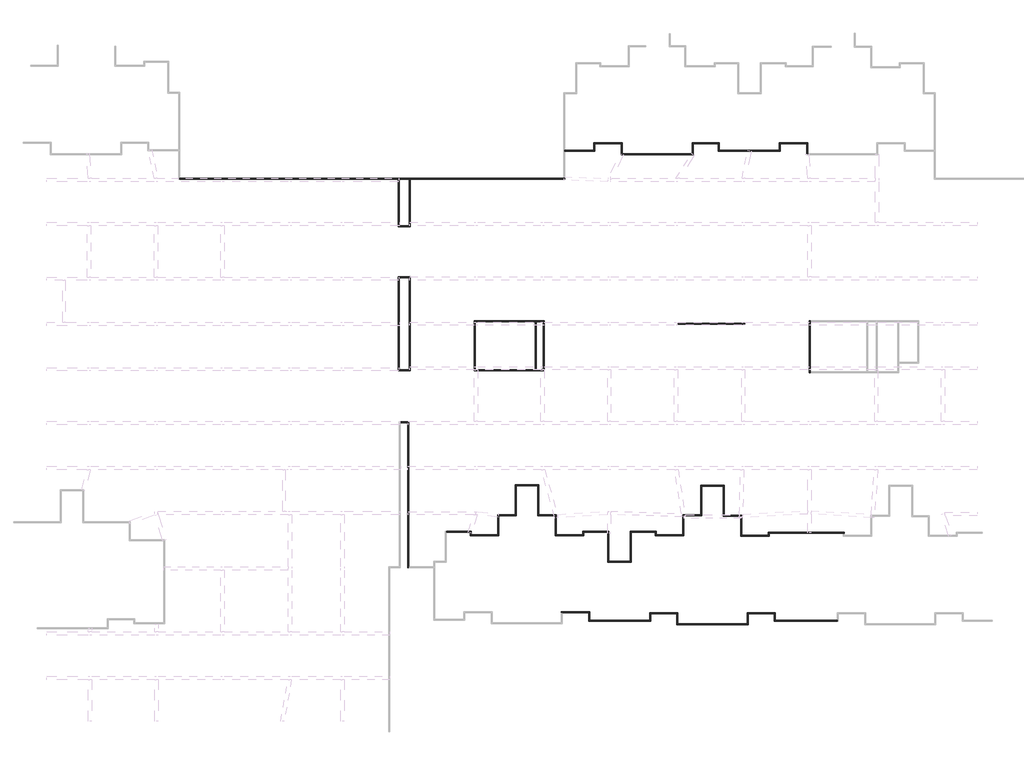
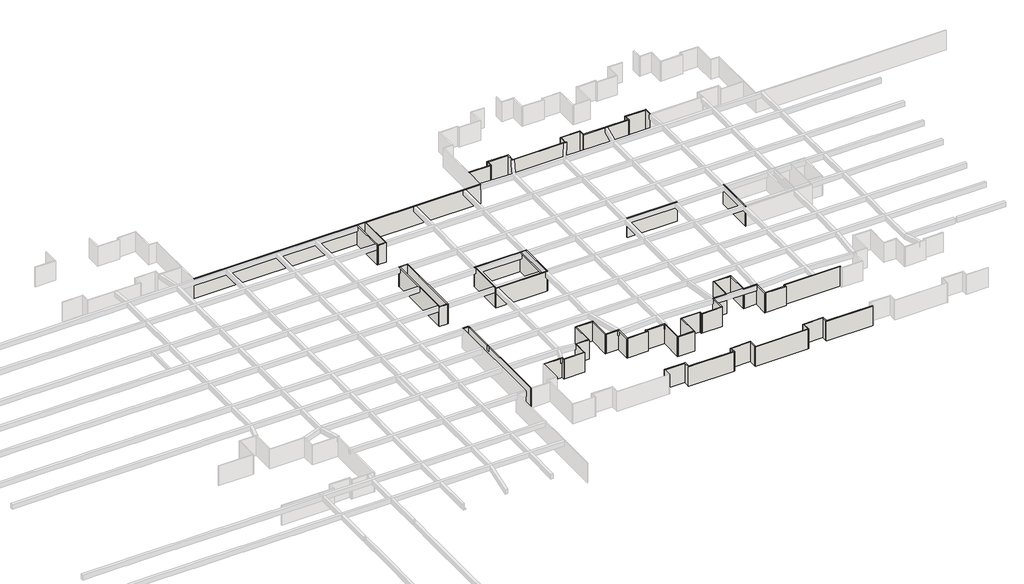
# One storey, part 5 of 16: 69 walls.
"""IFC4 building model written with IfcOpenShell, lengths in millimetres."""

from ifc_helpers import new_model, si_unit, origin, origin_with_axes, place, context, project, spatial, polyline, outline, extrude, faceted_brep, element, save

model = new_model("IFC4")

# Units and contexts
model_context = context("Model", 3, world=origin())
ifc_project = project(units=[si_unit("LENGTHUNIT", "METRE", prefix="MILLI")], contexts=[model_context])

# Site, building, storey
site = spatial("IfcSite", under=ifc_project)
building = spatial("IfcBuilding", under=site)
storey = spatial("IfcBuildingStorey", under=building, Name="户型图", Elevation=0.0)

# Walls
placement = place(None, origin())
element("IfcWall", 1, ObjectType="所有墙体", at=placement, inside=storey, context=model_context, shape_type="Brep", body=[
    faceted_brep([(305726.5285699, -132365.1471774, 0.0), (331943.757676, -132365.1471774, 0.0), (332063.757676, -132365.1471774, 0.0), (333243.7576761, -132365.1471774, 0.0), (333363.7576761, -132365.1471774, 0.0), (351926.5285699, -132365.1471774, 0.0), (351926.5285699, -132365.1471774, 3300.0), (333363.7576761, -132365.1471774, 3300.0), (333243.7576761, -132365.1471774, 3300.0), (332063.757676, -132365.1471774, 3300.0), (331943.757676, -132365.1471774, 3300.0), (305726.5285699, -132365.1471774, 3300.0), (305726.5285699, -132245.1471774, 0.0), (305726.5285699, -132245.1471774, 3300.0), (351806.5285699, -132245.1471774, 3300.0), (351926.5285699, -132245.1471774, 3300.0), (351926.5285699, -132245.1471774, 0.0), (351806.5285699, -132245.1471774, 0.0)], [[[0, 1, 2, 3, 4, 5, 6, 7, 8, 9, 10, 11]], [[12, 13, 14, 15, 16, 17]], [[5, 4, 3, 2, 1, 0, 12, 17, 16]], [[11, 10, 9, 8, 7, 6, 15, 14, 13]], [[0, 11, 13, 12]], [[6, 5, 16, 15]]]),
])
element("IfcWall", 2, ObjectType="所有墙体", at=placement, inside=storey, context=model_context, shape_type="Brep", body=[
    faceted_brep([(381017.0370116, -129335.4591871, 0.0), (381017.0370116, -128039.1416737, 0.0), (381017.0370116, -128039.1416737, 3300.0), (381017.0370116, -129335.4591871, 3300.0), (380897.0370116, -129335.4591871, 0.0), (380897.0370116, -129335.4591871, 3300.0), (380897.0370116, -128159.1416737, 3300.0), (380897.0370116, -128039.1416737, 3300.0), (380897.0370116, -128039.1416737, 0.0), (380897.0370116, -128159.1416737, 0.0)], [[[0, 1, 2, 3]], [[4, 5, 6, 7, 8, 9]], [[1, 0, 4, 9, 8]], [[3, 2, 7, 6, 5]], [[0, 3, 5, 4]], [[2, 1, 8, 7]]]),
])
element("IfcWall", 3, ObjectType="所有墙体", at=placement, inside=storey, context=model_context, shape_type="Brep", body=[
    faceted_brep([(380897.0370116, -128039.1416737, 0.0), (377598.9141674, -128039.1416737, 0.0), (377598.9141674, -128039.1416737, 3300.0), (380897.0370116, -128039.1416737, 3300.0), (380897.0370116, -128159.1416737, 0.0), (380897.0370116, -128159.1416737, 3300.0), (377718.9141674, -128159.1416737, 3300.0), (377598.9141674, -128159.1416737, 3300.0), (377598.9141674, -128159.1416737, 0.0), (377718.9141674, -128159.1416737, 0.0)], [[[0, 1, 2, 3]], [[4, 5, 6, 7, 8, 9]], [[1, 0, 4, 9, 8]], [[3, 2, 7, 6, 5]], [[0, 3, 5, 4]], [[2, 1, 8, 7]]]),
])
element("IfcWall", 4, ObjectType="所有墙体", at=placement, inside=storey, context=model_context, shape_type="Brep", body=[
    faceted_brep([(377598.9141674, -128159.1416737, 0.0), (377598.9141674, -128941.8026441, 0.0), (377598.9141674, -129061.8026441, 0.0), (377598.9141674, -129061.8026441, 3300.0), (377598.9141674, -128941.8026441, 3300.0), (377598.9141674, -128159.1416737, 3300.0), (377718.9141674, -128159.1416737, 0.0), (377718.9141674, -128159.1416737, 3300.0), (377718.9141674, -129061.8026441, 3300.0), (377718.9141674, -129061.8026441, 0.0)], [[[0, 1, 2, 3, 4, 5]], [[6, 7, 8, 9]], [[2, 1, 0, 6, 9]], [[5, 4, 3, 8, 7]], [[0, 5, 7, 6]], [[3, 2, 9, 8]]]),
])
element("IfcWall", 5, ObjectType="所有墙体", at=placement, inside=storey, context=model_context, shape_type="Brep", body=[
    faceted_brep([(377598.9141674, -128941.8026441, 0.0), (370417.9023455, -128941.8026441, 0.0), (370297.9023455, -128941.8026441, 0.0), (370297.9023455, -128941.8026441, 3300.0), (370417.9023455, -128941.8026441, 3300.0), (377598.9141674, -128941.8026441, 3300.0), (377598.9141674, -129061.8026441, 0.0), (377598.9141674, -129061.8026441, 3300.0), (370297.9023455, -129061.8026441, 3300.0), (370297.9023455, -129061.8026441, 0.0)], [[[0, 1, 2, 3, 4, 5]], [[6, 7, 8, 9]], [[2, 1, 0, 6, 9]], [[5, 4, 3, 8, 7]], [[0, 5, 7, 6]], [[3, 2, 9, 8]]]),
])
element("IfcWall", 6, ObjectType="所有墙体", at=placement, inside=storey, context=model_context, shape_type="Brep", body=[
    faceted_brep([(370417.9023455, -128941.8026441, 0.0), (370417.9023455, -128039.1416737, 0.0), (370417.9023455, -128039.1416737, 3300.0), (370417.9023455, -128941.8026441, 3300.0), (370297.9023455, -128941.8026441, 0.0), (370297.9023455, -128941.8026441, 3300.0), (370297.9023455, -128159.1416737, 3300.0), (370297.9023455, -128039.1416737, 3300.0), (370297.9023455, -128039.1416737, 0.0), (370297.9023455, -128159.1416737, 0.0)], [[[0, 1, 2, 3]], [[4, 5, 6, 7, 8, 9]], [[1, 0, 4, 9, 8]], [[3, 2, 7, 6, 5]], [[0, 3, 5, 4]], [[2, 1, 8, 7]]]),
])
element("IfcWall", 7, ObjectType="所有墙体", at=placement, inside=storey, context=model_context, shape_type="Brep", body=[
    faceted_brep([(370297.9023455, -128039.1416737, 0.0), (367198.9076923, -128039.1416737, 0.0), (367198.9076923, -128039.1416737, 3300.0), (370297.9023455, -128039.1416737, 3300.0), (370297.9023455, -128159.1416737, 0.0), (370297.9023455, -128159.1416737, 3300.0), (367318.9076923, -128159.1416737, 3300.0), (367198.9076923, -128159.1416737, 3300.0), (367198.9076923, -128159.1416737, 0.0), (367318.9076923, -128159.1416737, 0.0)], [[[0, 1, 2, 3]], [[4, 5, 6, 7, 8, 9]], [[1, 0, 4, 9, 8]], [[3, 2, 7, 6, 5]], [[0, 3, 5, 4]], [[2, 1, 8, 7]]]),
])
element("IfcWall", 8, ObjectType="所有墙体", at=placement, inside=storey, context=model_context, shape_type="Brep", body=[
    faceted_brep([(367198.9076923, -128159.1416737, 0.0), (367198.9076923, -129335.4591871, 0.0), (367198.9076923, -129455.4591871, 0.0), (367198.9076923, -129455.4591871, 3300.0), (367198.9076923, -129335.4591871, 3300.0), (367198.9076923, -128159.1416737, 3300.0), (367318.9076923, -128159.1416737, 0.0), (367318.9076923, -128159.1416737, 3300.0), (367318.9076923, -129455.4591871, 3300.0), (367318.9076923, -129455.4591871, 0.0)], [[[0, 1, 2, 3, 4, 5]], [[6, 7, 8, 9]], [[2, 1, 0, 6, 9]], [[5, 4, 3, 8, 7]], [[0, 5, 7, 6]], [[3, 2, 9, 8]]]),
])
element("IfcWall", 9, ObjectType="所有墙体", at=placement, inside=storey, context=model_context, shape_type="Brep", body=[
    faceted_brep([(367198.9076923, -129335.4591871, 0.0), (358817.8429758, -129335.4591871, 0.0), (358697.8429758, -129335.4591871, 0.0), (358697.8429758, -129335.4591871, 3300.0), (358817.8429758, -129335.4591871, 3300.0), (367198.9076923, -129335.4591871, 3300.0), (367198.9076923, -129455.4591871, 0.0), (367198.9076923, -129455.4591871, 3300.0), (358697.8429758, -129455.4591871, 3300.0), (358697.8429758, -129455.4591871, 0.0)], [[[0, 1, 2, 3, 4, 5]], [[6, 7, 8, 9]], [[2, 1, 0, 6, 9]], [[5, 4, 3, 8, 7]], [[0, 5, 7, 6]], [[3, 2, 9, 8]]]),
])
element("IfcWall", 10, ObjectType="所有墙体", at=placement, inside=storey, context=model_context, shape_type="Brep", body=[
    faceted_brep([(358817.8429758, -129335.4591871, 0.0), (358817.8429758, -128039.1416737, 0.0), (358817.8429758, -128039.1416737, 3300.0), (358817.8429758, -129335.4591871, 3300.0), (358697.8429758, -129335.4591871, 0.0), (358697.8429758, -129335.4591871, 3300.0), (358697.8429758, -128159.1416737, 3300.0), (358697.8429758, -128039.1416737, 3300.0), (358697.8429758, -128039.1416737, 0.0), (358697.8429758, -128159.1416737, 0.0)], [[[0, 1, 2, 3]], [[4, 5, 6, 7, 8, 9]], [[1, 0, 4, 9, 8]], [[3, 2, 7, 6, 5]], [[0, 3, 5, 4]], [[2, 1, 8, 7]]]),
])
element("IfcWall", 11, ObjectType="所有墙体", at=placement, inside=storey, context=model_context, shape_type="Brep", body=[
    faceted_brep([(358697.8429758, -128039.1416737, 0.0), (355398.9003454, -128039.1416737, 0.0), (355398.9003454, -128039.1416737, 3300.0), (358697.8429758, -128039.1416737, 3300.0), (358697.8429758, -128159.1416737, 0.0), (358697.8429758, -128159.1416737, 3300.0), (355518.9003454, -128159.1416737, 3300.0), (355398.9003454, -128159.1416737, 3300.0), (355398.9003454, -128159.1416737, 0.0), (355518.9003454, -128159.1416737, 0.0)], [[[0, 1, 2, 3]], [[4, 5, 6, 7, 8, 9]], [[1, 0, 4, 9, 8]], [[3, 2, 7, 6, 5]], [[0, 3, 5, 4]], [[2, 1, 8, 7]]]),
])
element("IfcWall", 12, ObjectType="所有墙体", at=placement, inside=storey, context=model_context, shape_type="Brep", body=[
    faceted_brep([(355398.9003454, -128159.1416737, 0.0), (355398.9003454, -128941.8026441, 0.0), (355398.9003454, -129061.8026441, 0.0), (355398.9003454, -129061.8026441, 3300.0), (355398.9003454, -128941.8026441, 3300.0), (355398.9003454, -128159.1416737, 3300.0), (355518.9003454, -128159.1416737, 0.0), (355518.9003454, -128159.1416737, 3300.0), (355518.9003454, -129061.8026441, 3300.0), (355518.9003454, -129061.8026441, 0.0)], [[[0, 1, 2, 3, 4, 5]], [[6, 7, 8, 9]], [[2, 1, 0, 6, 9]], [[5, 4, 3, 8, 7]], [[0, 5, 7, 6]], [[3, 2, 9, 8]]]),
])
element("IfcWall", 13, ObjectType="所有墙体", at=placement, inside=storey, context=model_context, shape_type="SweptSolid", body=[
    extrude(outline(polyline([(351926.5285699, -128941.8026441), (355398.9003454, -128941.8026441), (355398.9003454, -129061.8026441), (351926.5285699, -129061.8026441), (351926.5285699, -128941.8026441)])), origin_with_axes(), (0.0, 0.0, 1.0), 3300.0),
])
element("IfcWall", 14, ObjectType="所有墙体", at=placement, inside=storey, context=model_context, shape_type="Brep", body=[
    faceted_brep([(384538.9658496, -185270.5257617, 0.0), (377116.6006772, -185270.5257617, 0.0), (376996.6006772, -185270.5257617, 0.0), (376996.6006772, -185270.5257617, 3300.0), (377116.6006772, -185270.5257617, 3300.0), (384538.9658496, -185270.5257617, 3300.0), (384538.9658496, -185390.5257617, 0.0), (384538.9658496, -185390.5257617, 3300.0), (376996.6006772, -185390.5257617, 3300.0), (376996.6006772, -185390.5257617, 0.0)], [[[0, 1, 2, 3, 4, 5]], [[6, 7, 8, 9]], [[2, 1, 0, 6, 9]], [[5, 4, 3, 8, 7]], [[0, 5, 7, 6]], [[3, 2, 9, 8]]]),
])
element("IfcWall", 15, ObjectType="所有墙体", at=placement, inside=storey, context=model_context, shape_type="Brep", body=[
    faceted_brep([(377116.6006772, -185270.5257617, 0.0), (377116.6006772, -184345.1471774, 0.0), (377116.6006772, -184345.1471774, 3300.0), (377116.6006772, -185270.5257617, 3300.0), (376996.6006772, -185270.5257617, 0.0), (376996.6006772, -185270.5257617, 3300.0), (376996.6006772, -184465.1471774, 3300.0), (376996.6006772, -184345.1471774, 3300.0), (376996.6006772, -184345.1471774, 0.0), (376996.6006772, -184465.1471774, 0.0)], [[[0, 1, 2, 3]], [[4, 5, 6, 7, 8, 9]], [[1, 0, 4, 9, 8]], [[3, 2, 7, 6, 5]], [[0, 3, 5, 4]], [[2, 1, 8, 7]]]),
])
element("IfcWall", 16, ObjectType="所有墙体", at=placement, inside=storey, context=model_context, shape_type="Brep", body=[
    faceted_brep([(376996.6006772, -184345.1471774, 0.0), (373798.9314816, -184345.1471774, 0.0), (373798.9314816, -184345.1471774, 3300.0), (376996.6006772, -184345.1471774, 3300.0), (376996.6006772, -184465.1471774, 0.0), (376996.6006772, -184465.1471774, 3300.0), (373918.9314816, -184465.1471774, 3300.0), (373798.9314816, -184465.1471774, 3300.0), (373798.9314816, -184465.1471774, 0.0), (373918.9314816, -184465.1471774, 0.0)], [[[0, 1, 2, 3]], [[4, 5, 6, 7, 8, 9]], [[1, 0, 4, 9, 8]], [[3, 2, 7, 6, 5]], [[0, 3, 5, 4]], [[2, 1, 8, 7]]]),
])
element("IfcWall", 17, ObjectType="所有墙体", at=placement, inside=storey, context=model_context, shape_type="Brep", body=[
    faceted_brep([(373798.9314816, -184465.1471774, 0.0), (373798.9314816, -185696.3013241, 0.0), (373798.9314816, -185816.3013241, 0.0), (373798.9314816, -185816.3013241, 3300.0), (373798.9314816, -185696.3013241, 3300.0), (373798.9314816, -184465.1471774, 3300.0), (373918.9314816, -184465.1471774, 0.0), (373918.9314816, -184465.1471774, 3300.0), (373918.9314816, -185816.3013241, 3300.0), (373918.9314816, -185816.3013241, 0.0)], [[[0, 1, 2, 3, 4, 5]], [[6, 7, 8, 9]], [[2, 1, 0, 6, 9]], [[5, 4, 3, 8, 7]], [[0, 5, 7, 6]], [[3, 2, 9, 8]]]),
])
element("IfcWall", 18, ObjectType="所有墙体", at=placement, inside=storey, context=model_context, shape_type="Brep", body=[
    faceted_brep([(373798.9314816, -185696.3013241, 0.0), (365418.9314816, -185696.3013241, 0.0), (365298.9314816, -185696.3013241, 0.0), (365298.9314816, -185696.3013241, 3300.0), (365418.9314816, -185696.3013241, 3300.0), (373798.9314816, -185696.3013241, 3300.0), (373798.9314816, -185816.3013241, 0.0), (373798.9314816, -185816.3013241, 3300.0), (365298.9314816, -185816.3013241, 3300.0), (365298.9314816, -185816.3013241, 0.0)], [[[0, 1, 2, 3, 4, 5]], [[6, 7, 8, 9]], [[2, 1, 0, 6, 9]], [[5, 4, 3, 8, 7]], [[0, 5, 7, 6]], [[3, 2, 9, 8]]]),
])
element("IfcWall", 19, ObjectType="所有墙体", at=placement, inside=storey, context=model_context, shape_type="Brep", body=[
    faceted_brep([(365418.9314816, -185696.3013241, 0.0), (365418.9314816, -184345.1471774, 0.0), (365418.9314816, -184345.1471774, 3300.0), (365418.9314816, -185696.3013241, 3300.0), (365298.9314816, -185696.3013241, 0.0), (365298.9314816, -185696.3013241, 3300.0), (365298.9314816, -184465.1471774, 3300.0), (365298.9314816, -184345.1471774, 3300.0), (365298.9314816, -184345.1471774, 0.0), (365298.9314816, -184465.1471774, 0.0)], [[[0, 1, 2, 3]], [[4, 5, 6, 7, 8, 9]], [[1, 0, 4, 9, 8]], [[3, 2, 7, 6, 5]], [[0, 3, 5, 4]], [[2, 1, 8, 7]]]),
])
element("IfcWall", 20, ObjectType="所有墙体", at=placement, inside=storey, context=model_context, shape_type="Brep", body=[
    faceted_brep([(365298.9314816, -184345.1471774, 0.0), (362098.9314816, -184345.1471774, 0.0), (362098.9314816, -184345.1471774, 3300.0), (365298.9314816, -184345.1471774, 3300.0), (365298.9314816, -184465.1471774, 0.0), (365298.9314816, -184465.1471774, 3300.0), (362218.9314816, -184465.1471774, 3300.0), (362098.9314816, -184465.1471774, 3300.0), (362098.9314816, -184465.1471774, 0.0), (362218.9314816, -184465.1471774, 0.0)], [[[0, 1, 2, 3]], [[4, 5, 6, 7, 8, 9]], [[1, 0, 4, 9, 8]], [[3, 2, 7, 6, 5]], [[0, 3, 5, 4]], [[2, 1, 8, 7]]]),
])
element("IfcWall", 21, ObjectType="所有墙体", at=placement, inside=storey, context=model_context, shape_type="Brep", body=[
    faceted_brep([(362098.9314816, -184465.1471774, 0.0), (362098.9314816, -185245.1471774, 0.0), (362098.9314816, -185365.1471774, 0.0), (362098.9314816, -185365.1471774, 3300.0), (362098.9314816, -185245.1471774, 3300.0), (362098.9314816, -184465.1471774, 3300.0), (362218.9314816, -184465.1471774, 0.0), (362218.9314816, -184465.1471774, 3300.0), (362218.9314816, -185365.1471774, 3300.0), (362218.9314816, -185365.1471774, 0.0)], [[[0, 1, 2, 3, 4, 5]], [[6, 7, 8, 9]], [[2, 1, 0, 6, 9]], [[5, 4, 3, 8, 7]], [[0, 5, 7, 6]], [[3, 2, 9, 8]]]),
])
element("IfcWall", 22, ObjectType="所有墙体", at=placement, inside=storey, context=model_context, shape_type="Brep", body=[
    faceted_brep([(362098.9314816, -185245.1471774, 0.0), (354918.9314816, -185245.1471774, 0.0), (354798.9314816, -185245.1471774, 0.0), (354798.9314816, -185245.1471774, 3300.0), (354918.9314816, -185245.1471774, 3300.0), (362098.9314816, -185245.1471774, 3300.0), (362098.9314816, -185365.1471774, 0.0), (362098.9314816, -185365.1471774, 3300.0), (354798.9314816, -185365.1471774, 3300.0), (354798.9314816, -185365.1471774, 0.0)], [[[0, 1, 2, 3, 4, 5]], [[6, 7, 8, 9]], [[2, 1, 0, 6, 9]], [[5, 4, 3, 8, 7]], [[0, 5, 7, 6]], [[3, 2, 9, 8]]]),
])
element("IfcWall", 23, ObjectType="所有墙体", at=placement, inside=storey, context=model_context, shape_type="Brep", body=[
    faceted_brep([(354918.9314816, -185245.1471774, 0.0), (354918.9314816, -184248.2301972, 0.0), (354918.9314816, -184248.2301972, 3300.0), (354918.9314816, -185245.1471774, 3300.0), (354798.9314816, -185245.1471774, 0.0), (354798.9314816, -185245.1471774, 3300.0), (354798.9314816, -184368.2301972, 3300.0), (354798.9314816, -184248.2301972, 3300.0), (354798.9314816, -184248.2301972, 0.0), (354798.9314816, -184368.2301972, 0.0)], [[[0, 1, 2, 3]], [[4, 5, 6, 7, 8, 9]], [[1, 0, 4, 9, 8]], [[3, 2, 7, 6, 5]], [[0, 3, 5, 4]], [[2, 1, 8, 7]]]),
])
element("IfcWall", 24, ObjectType="所有墙体", at=placement, inside=storey, context=model_context, shape_type="Brep", body=[
    faceted_brep([(354798.9314816, -184248.2301972, 0.0), (351498.9314816, -184248.2301972, 0.0), (351498.9314816, -184248.2301972, 3300.0), (354798.9314816, -184248.2301972, 3300.0), (354798.9314816, -184368.2301972, 0.0), (354798.9314816, -184368.2301972, 3300.0), (351618.9314816, -184368.2301972, 3300.0), (351498.9314816, -184368.2301972, 3300.0), (351498.9314816, -184368.2301972, 0.0), (351618.9314816, -184368.2301972, 0.0)], [[[0, 1, 2, 3]], [[4, 5, 6, 7, 8, 9]], [[1, 0, 4, 9, 8]], [[3, 2, 7, 6, 5]], [[0, 3, 5, 4]], [[2, 1, 8, 7]]]),
])
element("IfcWall", 25, ObjectType="所有墙体", at=placement, inside=storey, context=model_context, shape_type="Brep", body=[
    faceted_brep([(337684.3582015, -174724.5990482, 0.0), (340573.4669495, -174724.5990482, 0.0), (340693.4669495, -174724.5990482, 0.0), (340693.4669495, -174724.5990482, 3300.0), (340573.4669495, -174724.5990482, 3300.0), (337684.3582015, -174724.5990482, 3300.0), (337684.3582015, -174604.5990482, 0.0), (337684.3582015, -174604.5990482, 3300.0), (340693.4669495, -174604.5990482, 3300.0), (340693.4669495, -174604.5990482, 0.0)], [[[0, 1, 2, 3, 4, 5]], [[6, 7, 8, 9]], [[2, 1, 0, 6, 9]], [[5, 4, 3, 8, 7]], [[0, 5, 7, 6]], [[3, 2, 9, 8]]]),
])
element("IfcWall", 26, ObjectType="所有墙体", at=placement, inside=storey, context=model_context, shape_type="Brep", body=[
    faceted_brep([(340573.4669495, -174724.5990482, 0.0), (340573.4669495, -175132.2128424, 0.0), (340573.4669495, -175132.2128424, 3300.0), (340573.4669495, -174724.5990482, 3300.0), (340693.4669495, -174724.5990482, 0.0), (340693.4669495, -174724.5990482, 3300.0), (340693.4669495, -175012.2128424, 3300.0), (340693.4669495, -175132.2128424, 3300.0), (340693.4669495, -175132.2128424, 0.0), (340693.4669495, -175012.2128424, 0.0)], [[[0, 1, 2, 3]], [[4, 5, 6, 7, 8, 9]], [[1, 0, 4, 9, 8]], [[3, 2, 7, 6, 5]], [[0, 3, 5, 4]], [[2, 1, 8, 7]]]),
])
element("IfcWall", 27, ObjectType="所有墙体", at=placement, inside=storey, context=model_context, shape_type="Brep", body=[
    faceted_brep([(340693.4669495, -175132.2128424, 0.0), (343992.4463185, -175132.2128424, 0.0), (343992.4463185, -175132.2128424, 3300.0), (340693.4669495, -175132.2128424, 3300.0), (340693.4669495, -175012.2128424, 0.0), (340693.4669495, -175012.2128424, 3300.0), (343872.4463185, -175012.2128424, 3300.0), (343992.4463185, -175012.2128424, 3300.0), (343992.4463185, -175012.2128424, 0.0), (343872.4463185, -175012.2128424, 0.0)], [[[0, 1, 2, 3]], [[4, 5, 6, 7, 8, 9]], [[1, 0, 4, 9, 8]], [[3, 2, 7, 6, 5]], [[0, 3, 5, 4]], [[2, 1, 8, 7]]]),
])
element("IfcWall", 28, ObjectType="所有墙体", at=placement, inside=storey, context=model_context, shape_type="Brep", body=[
    faceted_brep([(343992.4463185, -175012.2128424, 0.0), (343992.4463185, -172740.550998, 0.0), (343992.4463185, -172620.550998, 0.0), (343992.4463185, -172620.550998, 3300.0), (343992.4463185, -172740.550998, 3300.0), (343992.4463185, -175012.2128424, 3300.0), (343872.4463185, -175012.2128424, 0.0), (343872.4463185, -175012.2128424, 3300.0), (343872.4463185, -172620.550998, 3300.0), (343872.4463185, -172620.550998, 0.0)], [[[0, 1, 2, 3, 4, 5]], [[6, 7, 8, 9]], [[2, 1, 0, 6, 9]], [[5, 4, 3, 8, 7]], [[0, 5, 7, 6]], [[3, 2, 9, 8]]]),
])
element("IfcWall", 29, ObjectType="所有墙体", at=placement, inside=storey, context=model_context, shape_type="Brep", body=[
    faceted_brep([(343992.4463185, -172740.550998, 0.0), (346098.5035209, -172740.550998, 0.0), (346098.5035209, -172740.550998, 3300.0), (343992.4463185, -172740.550998, 3300.0), (343992.4463185, -172620.550998, 0.0), (343992.4463185, -172620.550998, 3300.0), (345978.5035209, -172620.550998, 3300.0), (346098.5035209, -172620.550998, 3300.0), (346098.5035209, -172620.550998, 0.0), (345978.5035209, -172620.550998, 0.0)], [[[0, 1, 2, 3]], [[4, 5, 6, 7, 8, 9]], [[1, 0, 4, 9, 8]], [[3, 2, 7, 6, 5]], [[0, 3, 5, 4]], [[2, 1, 8, 7]]]),
])
element("IfcWall", 30, ObjectType="所有墙体", at=placement, inside=storey, context=model_context, shape_type="Brep", body=[
    faceted_brep([(346098.5035209, -172620.550998, 0.0), (346098.5035209, -169145.867431, 0.0), (346098.5035209, -169025.867431, 0.0), (346098.5035209, -169025.867431, 3300.0), (346098.5035209, -169145.867431, 3300.0), (346098.5035209, -172620.550998, 3300.0), (345978.5035209, -172620.550998, 0.0), (345978.5035209, -172620.550998, 3300.0), (345978.5035209, -169025.867431, 3300.0), (345978.5035209, -169025.867431, 0.0)], [[[0, 1, 2, 3, 4, 5]], [[6, 7, 8, 9]], [[2, 1, 0, 6, 9]], [[5, 4, 3, 8, 7]], [[0, 5, 7, 6]], [[3, 2, 9, 8]]]),
])
element("IfcWall", 31, ObjectType="所有墙体", at=placement, inside=storey, context=model_context, shape_type="Brep", body=[
    faceted_brep([(346098.5035209, -169145.867431, 0.0), (348687.606076, -169145.867431, 0.0), (348807.606076, -169145.867431, 0.0), (348807.606076, -169145.867431, 3300.0), (348687.606076, -169145.867431, 3300.0), (346098.5035209, -169145.867431, 3300.0), (346098.5035209, -169025.867431, 0.0), (346098.5035209, -169025.867431, 3300.0), (348807.606076, -169025.867431, 3300.0), (348807.606076, -169025.867431, 0.0)], [[[0, 1, 2, 3, 4, 5]], [[6, 7, 8, 9]], [[2, 1, 0, 6, 9]], [[5, 4, 3, 8, 7]], [[0, 5, 7, 6]], [[3, 2, 9, 8]]]),
])
element("IfcWall", 32, ObjectType="所有墙体", at=placement, inside=storey, context=model_context, shape_type="Brep", body=[
    faceted_brep([(348687.606076, -169145.867431, 0.0), (348687.606076, -172740.550998, 0.0), (348687.606076, -172740.550998, 3300.0), (348687.606076, -169145.867431, 3300.0), (348807.606076, -169145.867431, 0.0), (348807.606076, -169145.867431, 3300.0), (348807.606076, -172620.550998, 3300.0), (348807.606076, -172740.550998, 3300.0), (348807.606076, -172740.550998, 0.0), (348807.606076, -172620.550998, 0.0)], [[[0, 1, 2, 3]], [[4, 5, 6, 7, 8, 9]], [[1, 0, 4, 9, 8]], [[3, 2, 7, 6, 5]], [[0, 3, 5, 4]], [[2, 1, 8, 7]]]),
])
element("IfcWall", 33, ObjectType="所有墙体", at=placement, inside=storey, context=model_context, shape_type="Brep", body=[
    faceted_brep([(348807.606076, -172740.550998, 0.0), (350778.5188809, -172740.550998, 0.0), (350898.5188809, -172740.550998, 0.0), (350898.5188809, -172740.550998, 3300.0), (350778.5188809, -172740.550998, 3300.0), (348807.606076, -172740.550998, 3300.0), (348807.606076, -172620.550998, 0.0), (348807.606076, -172620.550998, 3300.0), (350898.5188809, -172620.550998, 3300.0), (350898.5188809, -172620.550998, 0.0)], [[[0, 1, 2, 3, 4, 5]], [[6, 7, 8, 9]], [[2, 1, 0, 6, 9]], [[5, 4, 3, 8, 7]], [[0, 5, 7, 6]], [[3, 2, 9, 8]]]),
])
element("IfcWall", 34, ObjectType="所有墙体", at=placement, inside=storey, context=model_context, shape_type="Brep", body=[
    faceted_brep([(350778.5188809, -172740.550998, 0.0), (350778.5188809, -175132.2128424, 0.0), (350778.5188809, -175132.2128424, 3300.0), (350778.5188809, -172740.550998, 3300.0), (350898.5188809, -172740.550998, 0.0), (350898.5188809, -172740.550998, 3300.0), (350898.5188809, -175012.2128424, 3300.0), (350898.5188809, -175132.2128424, 3300.0), (350898.5188809, -175132.2128424, 0.0), (350898.5188809, -175012.2128424, 0.0)], [[[0, 1, 2, 3]], [[4, 5, 6, 7, 8, 9]], [[1, 0, 4, 9, 8]], [[3, 2, 7, 6, 5]], [[0, 3, 5, 4]], [[2, 1, 8, 7]]]),
])
element("IfcWall", 35, ObjectType="所有墙体", at=placement, inside=storey, context=model_context, shape_type="Brep", body=[
    faceted_brep([(350898.5188809, -175132.2128424, 0.0), (354192.4789585, -175132.2128424, 0.0), (354192.4789585, -175132.2128424, 3300.0), (350898.5188809, -175132.2128424, 3300.0), (350898.5188809, -175012.2128424, 0.0), (350898.5188809, -175012.2128424, 3300.0), (354072.4789585, -175012.2128424, 3300.0), (354192.4789585, -175012.2128424, 3300.0), (354192.4789585, -175012.2128424, 0.0), (354072.4789585, -175012.2128424, 0.0)], [[[0, 1, 2, 3]], [[4, 5, 6, 7, 8, 9]], [[1, 0, 4, 9, 8]], [[3, 2, 7, 6, 5]], [[0, 3, 5, 4]], [[2, 1, 8, 7]]]),
])
element("IfcWall", 36, ObjectType="所有墙体", at=placement, inside=storey, context=model_context, shape_type="Brep", body=[
    faceted_brep([(354192.4789585, -175012.2128424, 0.0), (354192.4789585, -174724.5990482, 0.0), (354192.4789585, -174604.5990482, 0.0), (354192.4789585, -174604.5990482, 3300.0), (354192.4789585, -174724.5990482, 3300.0), (354192.4789585, -175012.2128424, 3300.0), (354072.4789585, -175012.2128424, 0.0), (354072.4789585, -175012.2128424, 3300.0), (354072.4789585, -174604.5990482, 3300.0), (354072.4789585, -174604.5990482, 0.0)], [[[0, 1, 2, 3, 4, 5]], [[6, 7, 8, 9]], [[2, 1, 0, 6, 9]], [[5, 4, 3, 8, 7]], [[0, 5, 7, 6]], [[3, 2, 9, 8]]]),
])
element("IfcWall", 37, ObjectType="所有墙体", at=placement, inside=storey, context=model_context, shape_type="Brep", body=[
    faceted_brep([(354192.4789585, -174724.5990482, 0.0), (357073.5197495, -174724.5990482, 0.0), (357193.5197495, -174724.5990482, 0.0), (357193.5197495, -174724.5990482, 3300.0), (357073.5197495, -174724.5990482, 3300.0), (354192.4789585, -174724.5990482, 3300.0), (354192.4789585, -174604.5990482, 0.0), (354192.4789585, -174604.5990482, 3300.0), (357193.5197495, -174604.5990482, 3300.0), (357193.5197495, -174604.5990482, 0.0)], [[[0, 1, 2, 3, 4, 5]], [[6, 7, 8, 9]], [[2, 1, 0, 6, 9]], [[5, 4, 3, 8, 7]], [[0, 5, 7, 6]], [[3, 2, 9, 8]]]),
])
element("IfcWall", 38, ObjectType="所有墙体", at=placement, inside=storey, context=model_context, shape_type="Brep", body=[
    faceted_brep([(357073.5197495, -174724.5990482, 0.0), (357073.5197495, -178321.3511104, 0.0), (357073.5197495, -178321.3511104, 3300.0), (357073.5197495, -174724.5990482, 3300.0), (357193.5197495, -174724.5990482, 0.0), (357193.5197495, -174724.5990482, 3300.0), (357193.5197495, -178201.3511104, 3300.0), (357193.5197495, -178321.3511104, 3300.0), (357193.5197495, -178321.3511104, 0.0), (357193.5197495, -178201.3511104, 0.0)], [[[0, 1, 2, 3]], [[4, 5, 6, 7, 8, 9]], [[1, 0, 4, 9, 8]], [[3, 2, 7, 6, 5]], [[0, 3, 5, 4]], [[2, 1, 8, 7]]]),
])
element("IfcWall", 39, ObjectType="所有墙体", at=placement, inside=storey, context=model_context, shape_type="Brep", body=[
    faceted_brep([(357193.5197495, -178321.3511104, 0.0), (359884.4292415, -178321.3511104, 0.0), (359884.4292415, -178321.3511104, 3300.0), (357193.5197495, -178321.3511104, 3300.0), (357193.5197495, -178201.3511104, 0.0), (357193.5197495, -178201.3511104, 3300.0), (359764.4292415, -178201.3511104, 3300.0), (359884.4292415, -178201.3511104, 3300.0), (359884.4292415, -178201.3511104, 0.0), (359764.4292415, -178201.3511104, 0.0)], [[[0, 1, 2, 3]], [[4, 5, 6, 7, 8, 9]], [[1, 0, 4, 9, 8]], [[3, 2, 7, 6, 5]], [[0, 3, 5, 4]], [[2, 1, 8, 7]]]),
])
element("IfcWall", 40, ObjectType="所有墙体", at=placement, inside=storey, context=model_context, shape_type="Brep", body=[
    faceted_brep([(359884.4292415, -178201.3511104, 0.0), (359884.4292415, -174724.5990482, 0.0), (359884.4292415, -174604.5990482, 0.0), (359884.4292415, -174604.5990482, 3300.0), (359884.4292415, -174724.5990482, 3300.0), (359884.4292415, -178201.3511104, 3300.0), (359764.4292415, -178201.3511104, 0.0), (359764.4292415, -178201.3511104, 3300.0), (359764.4292415, -174604.5990482, 3300.0), (359764.4292415, -174604.5990482, 0.0)], [[[0, 1, 2, 3, 4, 5]], [[6, 7, 8, 9]], [[2, 1, 0, 6, 9]], [[5, 4, 3, 8, 7]], [[0, 5, 7, 6]], [[3, 2, 9, 8]]]),
])
element("IfcWall", 41, ObjectType="所有墙体", at=placement, inside=storey, context=model_context, shape_type="Brep", body=[
    faceted_brep([(359884.4292415, -174724.5990482, 0.0), (362773.5379895, -174724.5990482, 0.0), (362893.5379895, -174724.5990482, 0.0), (362893.5379895, -174724.5990482, 3300.0), (362773.5379895, -174724.5990482, 3300.0), (359884.4292415, -174724.5990482, 3300.0), (359884.4292415, -174604.5990482, 0.0), (359884.4292415, -174604.5990482, 3300.0), (362893.5379895, -174604.5990482, 3300.0), (362893.5379895, -174604.5990482, 0.0)], [[[0, 1, 2, 3, 4, 5]], [[6, 7, 8, 9]], [[2, 1, 0, 6, 9]], [[5, 4, 3, 8, 7]], [[0, 5, 7, 6]], [[3, 2, 9, 8]]]),
])
element("IfcWall", 42, ObjectType="所有墙体", at=placement, inside=storey, context=model_context, shape_type="Brep", body=[
    faceted_brep([(362773.5379895, -174724.5990482, 0.0), (362773.5379895, -175124.5990482, 0.0), (362773.5379895, -175124.5990482, 3300.0), (362773.5379895, -174724.5990482, 3300.0), (362893.5379895, -174724.5990482, 0.0), (362893.5379895, -174724.5990482, 3300.0), (362893.5379895, -175004.5990482, 3300.0), (362893.5379895, -175124.5990482, 3300.0), (362893.5379895, -175124.5990482, 0.0), (362893.5379895, -175004.5990482, 0.0)], [[[0, 1, 2, 3]], [[4, 5, 6, 7, 8, 9]], [[1, 0, 4, 9, 8]], [[3, 2, 7, 6, 5]], [[0, 3, 5, 4]], [[2, 1, 8, 7]]]),
])
element("IfcWall", 43, ObjectType="所有墙体", at=placement, inside=storey, context=model_context, shape_type="Brep", body=[
    faceted_brep([(362893.5379895, -175124.5990482, 0.0), (366192.53662, -175124.5990482, 0.0), (366192.53662, -175124.5990482, 3300.0), (362893.5379895, -175124.5990482, 3300.0), (362893.5379895, -175004.5990482, 0.0), (362893.5379895, -175004.5990482, 3300.0), (366072.53662, -175004.5990482, 3300.0), (366192.53662, -175004.5990482, 3300.0), (366192.53662, -175004.5990482, 0.0), (366072.53662, -175004.5990482, 0.0)], [[[0, 1, 2, 3]], [[4, 5, 6, 7, 8, 9]], [[1, 0, 4, 9, 8]], [[3, 2, 7, 6, 5]], [[0, 3, 5, 4]], [[2, 1, 8, 7]]]),
])
element("IfcWall", 44, ObjectType="所有墙体", at=placement, inside=storey, context=model_context, shape_type="Brep", body=[
    faceted_brep([(366192.53662, -175004.5990482, 0.0), (366192.53662, -172724.5990482, 0.0), (366192.53662, -172604.5990482, 0.0), (366192.53662, -172604.5990482, 3300.0), (366192.53662, -172724.5990482, 3300.0), (366192.53662, -175004.5990482, 3300.0), (366072.53662, -175004.5990482, 0.0), (366072.53662, -175004.5990482, 3300.0), (366072.53662, -172604.5990482, 3300.0), (366072.53662, -172604.5990482, 0.0)], [[[0, 1, 2, 3, 4, 5]], [[6, 7, 8, 9]], [[2, 1, 0, 6, 9]], [[5, 4, 3, 8, 7]], [[0, 5, 7, 6]], [[3, 2, 9, 8]]]),
])
element("IfcWall", 45, ObjectType="所有墙体", at=placement, inside=storey, context=model_context, shape_type="Brep", body=[
    faceted_brep([(366192.53662, -172724.5990482, 0.0), (368298.6149165, -172724.5990482, 0.0), (368298.6149165, -172724.5990482, 3300.0), (366192.53662, -172724.5990482, 3300.0), (366192.53662, -172604.5990482, 0.0), (366192.53662, -172604.5990482, 3300.0), (368178.6149165, -172604.5990482, 3300.0), (368298.6149165, -172604.5990482, 3300.0), (368298.6149165, -172604.5990482, 0.0), (368178.6149165, -172604.5990482, 0.0)], [[[0, 1, 2, 3]], [[4, 5, 6, 7, 8, 9]], [[1, 0, 4, 9, 8]], [[3, 2, 7, 6, 5]], [[0, 3, 5, 4]], [[2, 1, 8, 7]]]),
])
element("IfcWall", 46, ObjectType="所有墙体", at=placement, inside=storey, context=model_context, shape_type="Brep", body=[
    faceted_brep([(368298.6149165, -172604.5990482, 0.0), (368298.6149165, -169202.0297951, 0.0), (368298.6149165, -169082.0297951, 0.0), (368298.6149165, -169082.0297951, 3300.0), (368298.6149165, -169202.0297951, 3300.0), (368298.6149165, -172604.5990482, 3300.0), (368178.6149165, -172604.5990482, 0.0), (368178.6149165, -172604.5990482, 3300.0), (368178.6149165, -169082.0297951, 3300.0), (368178.6149165, -169082.0297951, 0.0)], [[[0, 1, 2, 3, 4, 5]], [[6, 7, 8, 9]], [[2, 1, 0, 6, 9]], [[5, 4, 3, 8, 7]], [[0, 5, 7, 6]], [[3, 2, 9, 8]]]),
])
element("IfcWall", 47, ObjectType="所有墙体", at=placement, inside=storey, context=model_context, shape_type="Brep", body=[
    faceted_brep([(368298.6149165, -169202.0297951, 0.0), (370887.5350349, -169202.0297951, 0.0), (371007.5350349, -169202.0297951, 0.0), (371007.5350349, -169202.0297951, 3300.0), (370887.5350349, -169202.0297951, 3300.0), (368298.6149165, -169202.0297951, 3300.0), (368298.6149165, -169082.0297951, 0.0), (368298.6149165, -169082.0297951, 3300.0), (371007.5350349, -169082.0297951, 3300.0), (371007.5350349, -169082.0297951, 0.0)], [[[0, 1, 2, 3, 4, 5]], [[6, 7, 8, 9]], [[2, 1, 0, 6, 9]], [[5, 4, 3, 8, 7]], [[0, 5, 7, 6]], [[3, 2, 9, 8]]]),
])
element("IfcWall", 48, ObjectType="所有墙体", at=placement, inside=storey, context=model_context, shape_type="Brep", body=[
    faceted_brep([(370887.5350349, -169202.0297951, 0.0), (370887.5350349, -172802.0297951, 0.0), (370887.5350349, -172802.0297951, 3300.0), (370887.5350349, -169202.0297951, 3300.0), (371007.5350349, -169202.0297951, 0.0), (371007.5350349, -169202.0297951, 3300.0), (371007.5350349, -172682.0297951, 3300.0), (371007.5350349, -172802.0297951, 3300.0), (371007.5350349, -172802.0297951, 0.0), (371007.5350349, -172682.0297951, 0.0)], [[[0, 1, 2, 3]], [[4, 5, 6, 7, 8, 9]], [[1, 0, 4, 9, 8]], [[3, 2, 7, 6, 5]], [[0, 3, 5, 4]], [[2, 1, 8, 7]]]),
])
element("IfcWall", 49, ObjectType="所有墙体", at=placement, inside=storey, context=model_context, shape_type="Brep", body=[
    faceted_brep([(371007.5350349, -172802.0297951, 0.0), (372978.4343904, -172802.0297951, 0.0), (373098.4343904, -172802.0297951, 0.0), (373098.4343904, -172802.0297951, 3300.0), (372978.4343904, -172802.0297951, 3300.0), (371007.5350349, -172802.0297951, 3300.0), (371007.5350349, -172682.0297951, 0.0), (371007.5350349, -172682.0297951, 3300.0), (373098.4343904, -172682.0297951, 3300.0), (373098.4343904, -172682.0297951, 0.0)], [[[0, 1, 2, 3, 4, 5]], [[6, 7, 8, 9]], [[2, 1, 0, 6, 9]], [[5, 4, 3, 8, 7]], [[0, 5, 7, 6]], [[3, 2, 9, 8]]]),
])
element("IfcWall", 50, ObjectType="所有墙体", at=placement, inside=storey, context=model_context, shape_type="Brep", body=[
    faceted_brep([(372978.4343904, -172802.0297951, 0.0), (372978.4343904, -175202.0297951, 0.0), (372978.4343904, -175202.0297951, 3300.0), (372978.4343904, -172802.0297951, 3300.0), (373098.4343904, -172802.0297951, 0.0), (373098.4343904, -172802.0297951, 3300.0), (373098.4343904, -175082.0297951, 3300.0), (373098.4343904, -175202.0297951, 3300.0), (373098.4343904, -175202.0297951, 0.0), (373098.4343904, -175082.0297951, 0.0)], [[[0, 1, 2, 3]], [[4, 5, 6, 7, 8, 9]], [[1, 0, 4, 9, 8]], [[3, 2, 7, 6, 5]], [[0, 3, 5, 4]], [[2, 1, 8, 7]]]),
])
element("IfcWall", 51, ObjectType="所有墙体", at=placement, inside=storey, context=model_context, shape_type="Brep", body=[
    faceted_brep([(373098.4343904, -175202.0297951, 0.0), (376398.4343904, -175202.0297951, 0.0), (376398.4343904, -175202.0297951, 3300.0), (373098.4343904, -175202.0297951, 3300.0), (373098.4343904, -175082.0297951, 0.0), (373098.4343904, -175082.0297951, 3300.0), (376278.4343904, -175082.0297951, 3300.0), (376398.4343904, -175082.0297951, 3300.0), (376398.4343904, -175082.0297951, 0.0), (376278.4343904, -175082.0297951, 0.0)], [[[0, 1, 2, 3]], [[4, 5, 6, 7, 8, 9]], [[1, 0, 4, 9, 8]], [[3, 2, 7, 6, 5]], [[0, 3, 5, 4]], [[2, 1, 8, 7]]]),
])
element("IfcWall", 52, ObjectType="所有墙体", at=placement, inside=storey, context=model_context, shape_type="Brep", body=[
    faceted_brep([(376398.4343904, -175082.0297951, 0.0), (376398.4343904, -174822.5388289, 0.0), (376398.4343904, -174702.5388289, 0.0), (376398.4343904, -174702.5388289, 3300.0), (376398.4343904, -174822.5388289, 3300.0), (376398.4343904, -175082.0297951, 3300.0), (376278.4343904, -175082.0297951, 0.0), (376278.4343904, -175082.0297951, 3300.0), (376278.4343904, -174702.5388289, 3300.0), (376278.4343904, -174702.5388289, 0.0)], [[[0, 1, 2, 3, 4, 5]], [[6, 7, 8, 9]], [[2, 1, 0, 6, 9]], [[5, 4, 3, 8, 7]], [[0, 5, 7, 6]], [[3, 2, 9, 8]]]),
])
element("IfcWall", 53, ObjectType="所有墙体", at=placement, inside=storey, context=model_context, shape_type="Brep", body=[
    faceted_brep([(376398.4343904, -174822.5388289, 0.0), (385313.3623471, -174822.5388289, 0.0), (385433.3623471, -174822.5388289, 0.0), (385433.3623471, -174822.5388289, 3300.0), (385313.3623471, -174822.5388289, 3300.0), (376398.4343904, -174822.5388289, 3300.0), (376398.4343904, -174702.5388289, 0.0), (376398.4343904, -174702.5388289, 3300.0), (385433.3623471, -174702.5388289, 3300.0), (385433.3623471, -174702.5388289, 0.0)], [[[0, 1, 2, 3, 4, 5]], [[6, 7, 8, 9]], [[2, 1, 0, 6, 9]], [[5, 4, 3, 8, 7]], [[0, 5, 7, 6]], [[3, 2, 9, 8]]]),
])
element("IfcWall", 54, ObjectType="所有墙体", at=placement, inside=storey, context=model_context, shape_type="Brep", body=[
    faceted_brep([(332213.7576761, -161565.1471774, 0.0), (333093.7576761, -161565.1471774, 0.0), (333213.7576761, -161565.1471774, 0.0), (333213.7576761, -161565.1471774, 3300.0), (333093.7576761, -161565.1471774, 3300.0), (332213.7576761, -161565.1471774, 3300.0), (332213.7576761, -161445.1471774, 0.0), (332213.7576761, -161445.1471774, 3300.0), (333213.7576761, -161445.1471774, 3300.0), (333213.7576761, -161445.1471774, 0.0)], [[[0, 1, 2, 3, 4, 5]], [[6, 7, 8, 9]], [[2, 1, 0, 6, 9]], [[5, 4, 3, 8, 7]], [[0, 5, 7, 6]], [[3, 2, 9, 8]]]),
])
element("IfcWall", 55, ObjectType="所有墙体", at=placement, inside=storey, context=model_context, shape_type="Brep", body=[
    faceted_brep([(333093.7576761, -161565.1471774, 0.0), (333093.7576761, -178965.1471774, 0.0), (333093.7576761, -178965.1471774, 3300.0), (333093.7576761, -161565.1471774, 3300.0), (333213.7576761, -161565.1471774, 0.0), (333213.7576761, -161565.1471774, 3300.0), (333213.7576761, -178845.1471774, 3300.0), (333213.7576761, -178965.1471774, 3300.0), (333213.7576761, -178965.1471774, 0.0), (333213.7576761, -178845.1471774, 0.0)], [[[0, 1, 2, 3]], [[4, 5, 6, 7, 8, 9]], [[1, 0, 4, 9, 8]], [[3, 2, 7, 6, 5]], [[0, 3, 5, 4]], [[2, 1, 8, 7]]]),
])
element("IfcWall", 56, ObjectType="所有墙体", at=placement, inside=storey, context=model_context, shape_type="Brep", body=[
    faceted_brep([(331943.757676, -132365.1471774, 0.0), (331943.757676, -138065.1471774, 0.0), (331943.757676, -138065.1471774, 3300.0), (331943.757676, -132365.1471774, 3300.0), (332063.757676, -132365.1471774, 0.0), (332063.757676, -132365.1471774, 3300.0), (332063.757676, -137945.1471774, 3300.0), (332063.757676, -138065.1471774, 3300.0), (332063.757676, -138065.1471774, 0.0), (332063.757676, -137945.1471774, 0.0)], [[[0, 1, 2, 3]], [[4, 5, 6, 7, 8, 9]], [[1, 0, 4, 9, 8]], [[3, 2, 7, 6, 5]], [[0, 3, 5, 4]], [[2, 1, 8, 7]]]),
])
element("IfcWall", 57, ObjectType="所有墙体", at=placement, inside=storey, context=model_context, shape_type="Brep", body=[
    faceted_brep([(332063.757676, -138065.1471774, 0.0), (333363.7576761, -138065.1471774, 0.0), (333363.7576761, -138065.1471774, 3300.0), (332063.757676, -138065.1471774, 3300.0), (332063.757676, -137945.1471774, 0.0), (332063.757676, -137945.1471774, 3300.0), (333243.7576761, -137945.1471774, 3300.0), (333363.7576761, -137945.1471774, 3300.0), (333363.7576761, -137945.1471774, 0.0), (333243.7576761, -137945.1471774, 0.0)], [[[0, 1, 2, 3]], [[4, 5, 6, 7, 8, 9]], [[1, 0, 4, 9, 8]], [[3, 2, 7, 6, 5]], [[0, 3, 5, 4]], [[2, 1, 8, 7]]]),
])
element("IfcWall", 58, ObjectType="所有墙体", at=placement, inside=storey, context=model_context, shape_type="SweptSolid", body=[
    extrude(outline(polyline([(333363.7576761, -132365.1471774), (333363.7576761, -137945.1471774), (333243.7576761, -137945.1471774), (333243.7576761, -132365.1471774), (333363.7576761, -132365.1471774)])), origin_with_axes(), (0.0, 0.0, 1.0), 3300.0),
])
element("IfcWall", 59, ObjectType="所有墙体", at=placement, inside=storey, context=model_context, shape_type="Brep", body=[
    faceted_brep([(331943.7576761, -144185.7214763, 0.0), (332063.7576761, -144185.7214763, 0.0), (333243.7576761, -144185.7214763, 0.0), (333363.7576761, -144185.7214763, 0.0), (333363.7576761, -144185.7214763, 3300.0), (333243.7576761, -144185.7214763, 3300.0), (332063.7576761, -144185.7214763, 3300.0), (331943.7576761, -144185.7214763, 3300.0), (331943.7576761, -144065.7214763, 0.0), (331943.7576761, -144065.7214763, 3300.0), (333363.7576761, -144065.7214763, 3300.0), (333363.7576761, -144065.7214763, 0.0)], [[[0, 1, 2, 3, 4, 5, 6, 7]], [[8, 9, 10, 11]], [[3, 2, 1, 0, 8, 11]], [[7, 6, 5, 4, 10, 9]], [[4, 3, 11, 10]], [[0, 7, 9, 8]]]),
])
element("IfcWall", 60, ObjectType="所有墙体", at=placement, inside=storey, context=model_context, shape_type="Brep", body=[
    faceted_brep([(333243.7576761, -144185.7214763, 0.0), (333243.7576761, -155245.1471774, 0.0), (333243.7576761, -155365.1471774, 0.0), (333243.7576761, -155365.1471774, 3300.0), (333243.7576761, -155245.1471774, 3300.0), (333243.7576761, -144185.7214763, 3300.0), (333363.7576761, -144185.7214763, 0.0), (333363.7576761, -144185.7214763, 3300.0), (333363.7576761, -155365.1471774, 3300.0), (333363.7576761, -155365.1471774, 0.0)], [[[0, 1, 2, 3, 4, 5]], [[6, 7, 8, 9]], [[2, 1, 0, 6, 9]], [[5, 4, 3, 8, 7]], [[0, 5, 7, 6]], [[3, 2, 9, 8]]]),
])
element("IfcWall", 61, ObjectType="所有墙体", at=placement, inside=storey, context=model_context, shape_type="Brep", body=[
    faceted_brep([(333243.7576761, -155245.1471774, 0.0), (332063.7576761, -155245.1471774, 0.0), (331943.7576761, -155245.1471774, 0.0), (331943.7576761, -155245.1471774, 3300.0), (332063.7576761, -155245.1471774, 3300.0), (333243.7576761, -155245.1471774, 3300.0), (333243.7576761, -155365.1471774, 0.0), (333243.7576761, -155365.1471774, 3300.0), (331943.7576761, -155365.1471774, 3300.0), (331943.7576761, -155365.1471774, 0.0)], [[[0, 1, 2, 3, 4, 5]], [[6, 7, 8, 9]], [[2, 1, 0, 6, 9]], [[5, 4, 3, 8, 7]], [[0, 5, 7, 6]], [[3, 2, 9, 8]]]),
])
element("IfcWall", 62, ObjectType="所有墙体", at=placement, inside=storey, context=model_context, shape_type="SweptSolid", body=[
    extrude(outline(polyline([(332063.7576761, -144185.7214763), (332063.7576761, -155245.1471774), (331943.7576761, -155245.1471774), (331943.7576761, -144185.7214763), (332063.7576761, -144185.7214763)])), origin_with_axes(), (0.0, 0.0, 1.0), 3300.0),
])
element("IfcWall", 63, ObjectType="所有墙体", at=placement, inside=storey, context=model_context, shape_type="Brep", body=[
    faceted_brep([(341033.3824612, -149465.1471774, 0.0), (341153.3824612, -149465.1471774, 0.0), (348393.757676, -149465.1471774, 0.0), (348513.757676, -149465.1471774, 0.0), (349318.757676, -149465.1471774, 0.0), (349438.757676, -149465.1471774, 0.0), (349438.757676, -149465.1471774, 3300.0), (349318.757676, -149465.1471774, 3300.0), (348513.757676, -149465.1471774, 3300.0), (348393.757676, -149465.1471774, 3300.0), (341153.3824612, -149465.1471774, 3300.0), (341033.3824612, -149465.1471774, 3300.0), (341033.3824612, -149345.1471774, 0.0), (341033.3824612, -149345.1471774, 3300.0), (349438.757676, -149345.1471774, 3300.0), (349438.757676, -149345.1471774, 0.0)], [[[0, 1, 2, 3, 4, 5, 6, 7, 8, 9, 10, 11]], [[12, 13, 14, 15]], [[5, 4, 3, 2, 1, 0, 12, 15]], [[11, 10, 9, 8, 7, 6, 14, 13]], [[6, 5, 15, 14]], [[0, 11, 13, 12]]]),
])
element("IfcWall", 64, ObjectType="所有墙体", at=placement, inside=storey, context=model_context, shape_type="Brep", body=[
    faceted_brep([(349318.757676, -149465.1471774, 0.0), (349318.757676, -155245.1471774, 0.0), (349318.757676, -155365.1471774, 0.0), (349318.757676, -155365.1471774, 3300.0), (349318.757676, -155245.1471774, 3300.0), (349318.757676, -149465.1471774, 3300.0), (349438.757676, -149465.1471774, 0.0), (349438.757676, -149465.1471774, 3300.0), (349438.757676, -155365.1471774, 3300.0), (349438.757676, -155365.1471774, 0.0)], [[[0, 1, 2, 3, 4, 5]], [[6, 7, 8, 9]], [[2, 1, 0, 6, 9]], [[5, 4, 3, 8, 7]], [[0, 5, 7, 6]], [[3, 2, 9, 8]]]),
])
element("IfcWall", 65, ObjectType="所有墙体", at=placement, inside=storey, context=model_context, shape_type="Brep", body=[
    faceted_brep([(349318.757676, -155245.1471774, 0.0), (348513.757676, -155245.1471774, 0.0), (348393.757676, -155245.1471774, 0.0), (341153.3824612, -155245.1471774, 0.0), (341033.3824612, -155245.1471774, 0.0), (341033.3824612, -155245.1471774, 3300.0), (341153.3824612, -155245.1471774, 3300.0), (348393.757676, -155245.1471774, 3300.0), (348513.757676, -155245.1471774, 3300.0), (349318.757676, -155245.1471774, 3300.0), (349318.757676, -155365.1471774, 0.0), (349318.757676, -155365.1471774, 3300.0), (341033.3824612, -155365.1471774, 3300.0), (341033.3824612, -155365.1471774, 0.0)], [[[0, 1, 2, 3, 4, 5, 6, 7, 8, 9]], [[10, 11, 12, 13]], [[4, 3, 2, 1, 0, 10, 13]], [[9, 8, 7, 6, 5, 12, 11]], [[0, 9, 11, 10]], [[5, 4, 13, 12]]]),
])
element("IfcWall", 66, ObjectType="所有墙体", at=placement, inside=storey, context=model_context, shape_type="SweptSolid", body=[
    extrude(outline(polyline([(341153.3824612, -149465.1471774), (341153.3824612, -155245.1471774), (341033.3824612, -155245.1471774), (341033.3824612, -149465.1471774), (341153.3824612, -149465.1471774)])), origin_with_axes(), (0.0, 0.0, 1.0), 3300.0),
])
element("IfcWall", 67, ObjectType="所有墙体", at=placement, inside=storey, context=model_context, shape_type="SweptSolid", body=[
    extrude(outline(polyline([(348393.757676, -155245.1471774), (348393.757676, -149465.1471774), (348513.757676, -149465.1471774), (348513.757676, -155245.1471774), (348393.757676, -155245.1471774)])), origin_with_axes(), (0.0, 0.0, 1.0), 3300.0),
])
element("IfcWall", 68, ObjectType="所有墙体", at=placement, inside=storey, context=model_context, shape_type="SweptSolid", body=[
    extrude(outline(polyline([(373503.757676, -149765.1471774), (365503.757676, -149765.1471774), (365503.757676, -149645.1471774), (373503.757676, -149645.1471774), (373503.757676, -149765.1471774)])), origin_with_axes(), (0.0, 0.0, 1.0), 3300.0),
])
element("IfcWall", 69, ObjectType="所有墙体", at=placement, inside=storey, context=model_context, shape_type="Brep", body=[
    faceted_brep([(381193.757676, -149345.1471774, 0.0), (381193.757676, -155565.1471774, 0.0), (381193.757676, -155565.1471774, 3300.0), (381193.757676, -149345.1471774, 3300.0), (381313.757676, -149345.1471774, 0.0), (381313.757676, -149345.1471774, 3300.0), (381313.757676, -149465.1471774, 3300.0), (381313.757676, -155445.1471774, 3300.0), (381313.757676, -155565.1471774, 3300.0), (381313.757676, -155565.1471774, 0.0), (381313.757676, -155445.1471774, 0.0), (381313.757676, -149465.1471774, 0.0)], [[[0, 1, 2, 3]], [[4, 5, 6, 7, 8, 9, 10, 11]], [[1, 0, 4, 11, 10, 9]], [[3, 2, 8, 7, 6, 5]], [[2, 1, 9, 8]], [[0, 3, 5, 4]]]),
])

save(model, "model.ifc")

# Revit data of these elements
# Type "所有墙体"
#   Layers, outside or top first: 120 mm "默认" (function 1)
# Elements 1, 2, 3, 4, 5, 6, 7, 8, 9, 10, 11, 12, 13, 14, 15, 16, 17, 18, 19, 20, 21, 22, 23, 24, 25, 26, 27, 28, 29, 30, 31, 32, 33, 34, 35, 36, 37, 38, 39, 40, 41, 42, 43, 44, 45, 46, 47, 48, 49, 50, 51, 52, 53, 54, 55, 56, 57, 58, 59, 60, 61, 62, 63, 64, 65, 66, 67, 68, 69 (IfcWall, "所有墙体")
#   Top Offset = 0 mm
#   Base Offset = 0 mm
#   wall height = 3300 mm
#   Phase Created = 新构造
#   Base Constraint = 户型图
#   Top Constraint = 层高
#   Materials on its faces: "默认"
# Materials
#   "默认": class "其他", colour RGB 192 192 192, transparency 0, Cost = 0
